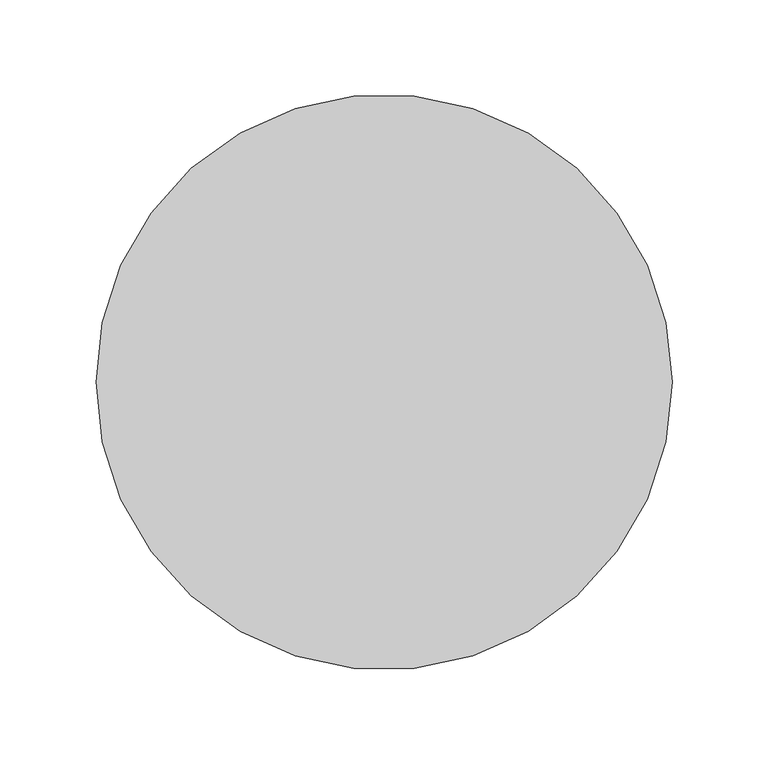
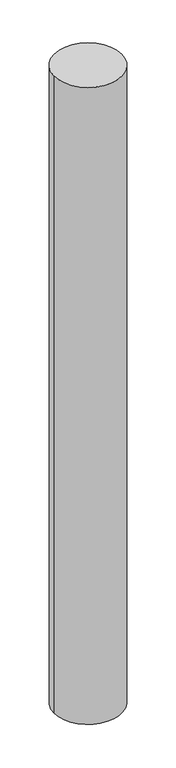
"""IFC4 building model written with IfcOpenShell, lengths in millimetres: column geometry, S-Column_CastInPlace_Round : Ø300."""

from ifc_helpers import new_model, si_unit, point, frame, origin, origin_2d, place, context, project, spatial, circle_curve, trimmed, segment, composite_curve, outline, extrude, source, transform, mapped, element, save


def column_70defcb8(model_context):
    return source(origin(), model_context, "Body", "SweptSolid", [
        extrude(outline(composite_curve([segment(trimmed(circle_curve(origin_2d(), 150.0), [point((-150.0, 0.0))], [point((150.0, 0.0))], False, "CARTESIAN"), True, "CONTINUOUS"), segment(trimmed(circle_curve(origin_2d(), 150.0), [point((150.0, 0.0))], [point((-150.0, 0.0))], False, "CARTESIAN"), True, "CONTINUOUS")], self_intersect=False)), frame((0.0, 0.0, -3000.0), z_axis=(0.0, 0.0, 1.0), x_axis=(1.0, 0.0, 0.0)), (0.0, 0.0, 1.0), 3000.0),
    ])


if __name__ == "__main__":
    model = new_model("IFC4")
    model_context = context("Model", 3, world=origin())
    ifc_project = project(units=[si_unit("LENGTHUNIT", "METRE", prefix="MILLI")], contexts=[model_context])
    site = spatial("IfcSite", under=ifc_project)
    building = spatial("IfcBuilding", under=site)
    placement = place(None, origin())
    column_shape = column_70defcb8(model_context)
    element("IfcColumn", 1, ObjectType="S-Column_CastInPlace_Round : Ø300", at=placement, inside=building, context=model_context, shape_type="MappedRepresentation", body=[
        mapped(column_shape, transform((0.0, 0.0, 0.0), x_axis=(1.0, 0.0, 0.0), y_axis=(0.0, 1.0, 0.0), z_axis=(0.0, 0.0, 1.0))),
    ])
    save(model, "model.ifc")

# Revit data of these elements
# Type "S-Column_CastInPlace_Round : Ø300"
#   NS3457-8 Code = "ASA"
#   NS3451 Code = "2220"
#   NS3457-8 = "ASA Konstruktive søyler"
#   NS3451 = "2220 Søyler"
#   Manufacturer = "Norconsult"
#   Description = "Plasstøpt"
#   Diameter = 300 mm
#   Structural Material = Concrete - Cast In Place
#   Assembly Code = ""
# Element 1 (IfcColumn, "S-Column_CastInPlace_Round : Ø300")
#   Materials on its faces: "Concrete - Cast In Place"
# Materials
#   "Concrete - Cast In Place": class "Concrete", colour RGB 186 186 186, transparency 0, Cost = 0
